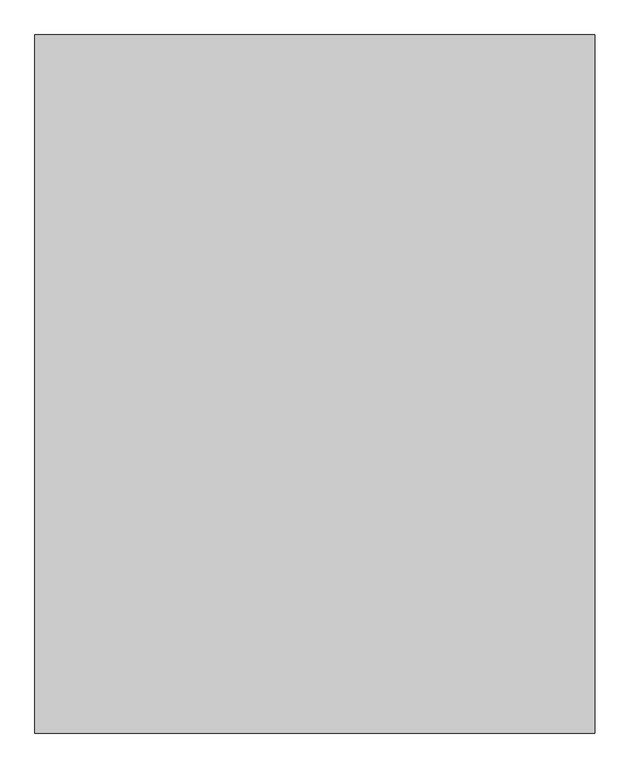
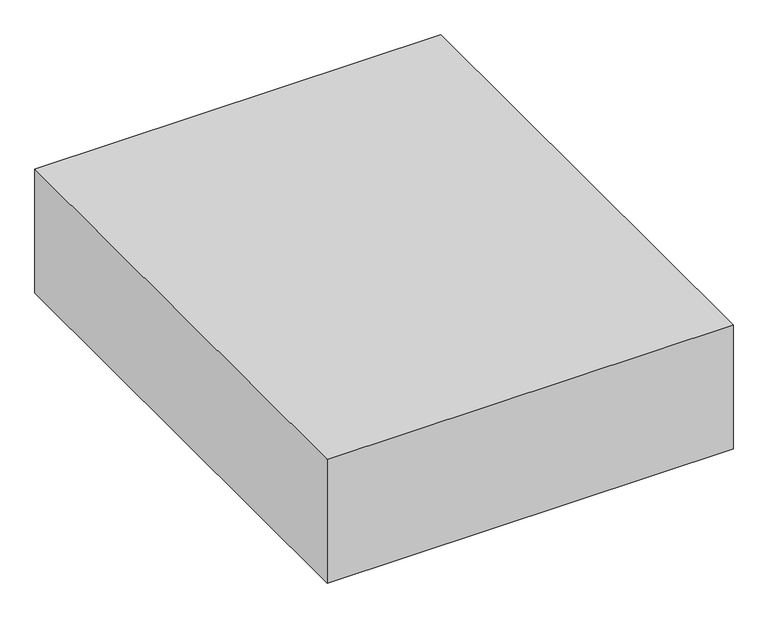
"""IFC4 building model written with IfcOpenShell, lengths in millimetres: proxy geometry, Space Planning Box_hec : Space Planning Box_hec."""

import ifcopenshell
import ifcopenshell.guid

model = None  # the IFC model being written
_history = None  # IfcOwnerHistory: only IFC2X3 demands one
_inside = {}  # id of a spatial element -> (the spatial element, [elements in it])
_under = {}  # id of a project, library or spatial element -> (it, [spatial elements below it])
_declared = {}  # id of a project -> (the project, [libraries it declares])
_typed = {}  # id of a type object -> (the type object, [elements of that type])
_made_of = {}  # id of a material, layer set ... -> (it, [elements and type objects made of it])


def new_model(schema):
    """Start an empty IFC model of exactly this schema.

    Asked for "IFC4X3", IfcOpenShell would pick the latest addendum, in which some entities
    have other attributes; the version numbers below select the first issue.
    IFC2X3 requires an IfcOwnerHistory on every rooted entity: one is made here for all.
    """
    global model, _history
    if schema == "IFC4X3":
        model = ifcopenshell.file(schema_version=(4, 3, 0, 0))
    else:
        model = ifcopenshell.file(schema=schema)
    _inside.clear()
    _under.clear()
    _declared.clear()
    _typed.clear()
    _made_of.clear()
    _history = None
    if model.schema == "IFC2X3":
        org = make("IfcOrganization", Name="unknown")
        user = make(
            "IfcPersonAndOrganization",
            ThePerson=make("IfcPerson", FamilyName="unknown"),
            TheOrganization=org,
        )
        app = make(
            "IfcApplication",
            ApplicationDeveloper=org,
            Version="unknown",
            ApplicationFullName="unknown",
            ApplicationIdentifier="unknown",
        )
        _history = make(
            "IfcOwnerHistory",
            OwningUser=user,
            OwningApplication=app,
            ChangeAction="ADDED",
            CreationDate=0,
        )
    return model


def make(cls, **values):
    """One entity of the class cls with the attributes given. An attribute that is None is left unset."""
    return model.create_entity(
        cls, **{name: value for name, value in values.items() if value is not None}
    )


def rooted(cls, **values):
    """An entity with a GlobalId (a new one), such as an element, a storey or a relation."""
    return make(cls, GlobalId=ifcopenshell.guid.new(), OwnerHistory=_history, **values)


def si_unit(unit_type, name, prefix=None):
    """IfcSIUnit, for example si_unit("LENGTHUNIT", "METRE", prefix="MILLI")."""
    return make("IfcSIUnit", UnitType=unit_type, Prefix=prefix, Name=name)


def assignment(units):
    """IfcUnitAssignment: the units of a project."""
    return None if units is None else make("IfcUnitAssignment", Units=units)


def point(xyz):
    """IfcCartesianPoint."""
    return None if xyz is None else make("IfcCartesianPoint", Coordinates=xyz)


def direction(xyz):
    """IfcDirection."""
    return None if xyz is None else make("IfcDirection", DirectionRatios=xyz)


def frame(location, z_axis=None, x_axis=None):
    """IfcAxis2Placement3D, a coordinate frame: its origin and axes. An axis left out is left unset."""
    return make(
        "IfcAxis2Placement3D",
        Location=point(location),
        Axis=direction(z_axis),
        RefDirection=direction(x_axis),
    )


def origin():
    """The frame at (0, 0, 0) with its axes left unset."""
    return frame((0.0, 0.0, 0.0))


def origin_with_axes():
    """The frame at (0, 0, 0) with the z axis (0, 0, 1) and the x axis (1, 0, 0) written out."""
    return frame((0.0, 0.0, 0.0), z_axis=(0.0, 0.0, 1.0), x_axis=(1.0, 0.0, 0.0))


def place(relative_to, where):
    """IfcLocalPlacement: puts the frame where relative to a parent placement (None: the world)."""
    return make(
        "IfcLocalPlacement", PlacementRelTo=relative_to, RelativePlacement=where
    )


def context(
    kind, dimensions, precision=None, world=None, true_north=None, identifier=None
):
    """IfcGeometricRepresentationContext, for example the 3D "Model" context."""
    return make(
        "IfcGeometricRepresentationContext",
        ContextIdentifier=identifier,
        ContextType=kind,
        CoordinateSpaceDimension=dimensions,
        Precision=precision,
        WorldCoordinateSystem=world,
        TrueNorth=true_north,
    )


def project(units=None, contexts=None):
    """IfcProject with its units and contexts."""
    return rooted(
        "IfcProject",
        Name="project",
        RepresentationContexts=contexts,
        UnitsInContext=assignment(units),
    )


def spatial(cls, under=None, at=None, **own):
    """A site, building, storey or space (cls), placed at a placement, below another one or the project."""
    s = rooted(cls, ObjectPlacement=at, **own)
    if under is not None:
        _under.setdefault(under.id(), (under, []))[1].append(s)
    return s


def polyline(points):
    """IfcPolyline through the points."""
    return make("IfcPolyline", Points=[point(p) for p in points])


def outline(outer, holes=None, kind="AREA"):
    """IfcArbitraryClosedProfileDef: a profile drawn as a closed curve; with holes, ...WithVoids."""
    if holes is None:
        return make("IfcArbitraryClosedProfileDef", ProfileType=kind, OuterCurve=outer)
    return make(
        "IfcArbitraryProfileDefWithVoids",
        ProfileType=kind,
        OuterCurve=outer,
        InnerCurves=holes,
    )


def extrude(swept, where, along, depth):
    """IfcExtrudedAreaSolid: the profile swept, set in the frame where, extruded along a direction by depth."""
    return make(
        "IfcExtrudedAreaSolid",
        SweptArea=swept,
        Position=where,
        ExtrudedDirection=direction(along),
        Depth=depth,
    )


def shape(context_of_items, identifier, shape_type, items):
    """IfcShapeRepresentation: the items that make up one representation, for example the "Body"."""
    return make(
        "IfcShapeRepresentation",
        ContextOfItems=context_of_items,
        RepresentationIdentifier=identifier,
        RepresentationType=shape_type,
        Items=items,
    )


def source(mapping_origin, context_of_items, identifier, shape_type, items):
    """IfcRepresentationMap: a shape defined once, which mapped items show again and again."""
    return make(
        "IfcRepresentationMap",
        MappingOrigin=mapping_origin,
        MappedRepresentation=shape(context_of_items, identifier, shape_type, items),
    )


def transform(
    local_origin,
    x_axis=None,
    y_axis=None,
    z_axis=None,
    scale=None,
    scale2=None,
    scale3=None,
    uniform=True,
):
    """IfcCartesianTransformationOperator3D, or its non-uniform kind. x_axis, y_axis, z_axis: its Axis1, 2, 3."""
    if uniform:
        return make(
            "IfcCartesianTransformationOperator3D",
            Axis1=direction(x_axis),
            Axis2=direction(y_axis),
            LocalOrigin=point(local_origin),
            Scale=scale,
            Axis3=direction(z_axis),
        )
    return make(
        "IfcCartesianTransformationOperator3DnonUniform",
        Axis1=direction(x_axis),
        Axis2=direction(y_axis),
        LocalOrigin=point(local_origin),
        Scale=scale,
        Axis3=direction(z_axis),
        Scale2=scale2,
        Scale3=scale3,
    )


def mapped(mapping_source, mapping_target):
    """IfcMappedItem: shows the shape of a source again, moved by a transform."""
    return make(
        "IfcMappedItem", MappingSource=mapping_source, MappingTarget=mapping_target
    )


def made_of(thing, what):
    """Note that an element or type object is made of a material, layer set ...; save() writes the relation."""
    if what is not None:
        _made_of.setdefault(what.id(), (what, []))[1].append(thing)
    return thing


def element(
    cls,
    number,
    at=None,
    inside=None,
    cuts=None,
    type_object=None,
    material=None,
    context=None,
    identifier="Body",
    shape_type=None,
    held_by="IfcProductDefinitionShape",
    body=None,
    shapes=None,
    **own,
):
    """One element of the class cls, such as IfcWall. Its Tag is "e" and its number.

    at: its placement. inside: the storey or other place that contains it. cuts: it is an
    opening in that element (IfcRelVoidsElement). A single representation is given by context,
    identifier, shape_type and body (its items); several are given by shapes. held_by: the class
    of the entity that holds the representations. save() writes the other relations.
    """
    e = rooted(cls, Tag="e%d" % number, ObjectPlacement=at, **own)
    if body is not None:
        shapes = [shape(context, identifier, shape_type, body)]
    if shapes is not None:
        e.Representation = make(held_by, Representations=shapes)
    if inside is not None:
        _inside.setdefault(inside.id(), (inside, []))[1].append(e)
    if cuts is not None:
        rooted(
            "IfcRelVoidsElement", RelatingBuildingElement=cuts, RelatedOpeningElement=e
        )
    if type_object is not None:
        _typed.setdefault(type_object.id(), (type_object, []))[1].append(e)
    return made_of(e, material)


def aggregate(whole, parts):
    """IfcRelAggregates: a whole, such as a stair, and the parts it consists of."""
    return rooted("IfcRelAggregates", RelatingObject=whole, RelatedObjects=parts)


def save(model, path):
    """Write the relations noted so far, then the file.

    IfcRelAggregates (storeys below a building ...), IfcRelContainedInSpatialStructure (elements
    in a storey), IfcRelDefinesByType, IfcRelAssociatesMaterial and IfcRelDeclares: one each for
    every whole, place, type object, material and project.
    """
    for whole, parts in _under.values():
        aggregate(whole, parts)
    for where, things in _inside.values():
        rooted(
            "IfcRelContainedInSpatialStructure",
            RelatedElements=things,
            RelatingStructure=where,
        )
    for kind, things in _typed.values():
        rooted("IfcRelDefinesByType", RelatedObjects=things, RelatingType=kind)
    for what, things in _made_of.values():
        rooted("IfcRelAssociatesMaterial", RelatedObjects=things, RelatingMaterial=what)
    for by, libraries in _declared.values():
        rooted("IfcRelDeclares", RelatingContext=by, RelatedDefinitions=libraries)
    model.write(path)


def generic_models_d82b1902(model_context):
    return source(origin(), model_context, "Body", "SweptSolid", [
        extrude(outline(polyline([(9300.0, 11600.0), (9300.0, -11600.0), (-9300.0, -11600.0), (-9300.0, 11600.0), (9300.0, 11600.0)])), origin_with_axes(), (0.0, 0.0, 1.0), 6000.0),
    ])


if __name__ == "__main__":
    model = new_model("IFC4")
    model_context = context("Model", 3, world=origin())
    ifc_project = project(units=[si_unit("LENGTHUNIT", "METRE", prefix="MILLI")], contexts=[model_context])
    site = spatial("IfcSite", under=ifc_project)
    building = spatial("IfcBuilding", under=site)
    placement = place(None, origin())
    generic_models_shape = generic_models_d82b1902(model_context)
    element("IfcBuildingElementProxy", 1, Name="Space Planning Box_hec : Space Planning Box_hec", ObjectType="Space Planning Box_hec : Space Planning Box_hec", at=placement, inside=building, context=model_context, shape_type="MappedRepresentation", body=[
        mapped(generic_models_shape, transform((0.0, 0.0, 0.0), x_axis=(1.0, 0.0, 0.0), y_axis=(0.0, 1.0, 0.0), z_axis=(0.0, 0.0, 1.0))),
    ])
    save(model, "model.ifc")

# Revit data of these elements
# Type "Space Planning Box_hec : Space Planning Box_hec"
#   Type Comments = "..."
#   Room Name [instance default] = "?"
#   Interior Finish [instance default] = ""
#   Exterior Finish [instance default] = ""
#   Department [instance default] = ""
#   Assembly Code = "..."
#   Width [instance default] = 1524 mm
#   Program Area [instance default] = 0.00 m²
#   Length [instance default] = 1524 mm
#   Height [instance default] = 1524 mm
#   Area [instance default] = 2.32258 m²
#   Fill Color [instance default] = Cyan
#   Default Elevation = 0
# Element 1 (IfcBuildingElementProxy, "Space Planning Box_hec : Space Planning Box_hec")
#   Room Name = "Electronic Room"
#   Interior Finish = "IF1"
#   Exterior Finish = "EF1"
#   Department = "CI"
#   Width = 18600 mm
#   Program Area = 431.52 m²
#   Length = 23200 mm
#   Height = 6000 mm
#   Area = 431.52 m²
#   Fill Color = Lime
#   Materials on its faces: "Lime"
# Materials
#   "Cyan": class "Generic", colour RGB 0 255 255, transparency 0.2, Cost = 0
#   "Lime": class "Generic", colour RGB 0 255 0, transparency 0.2, Cost = 0
